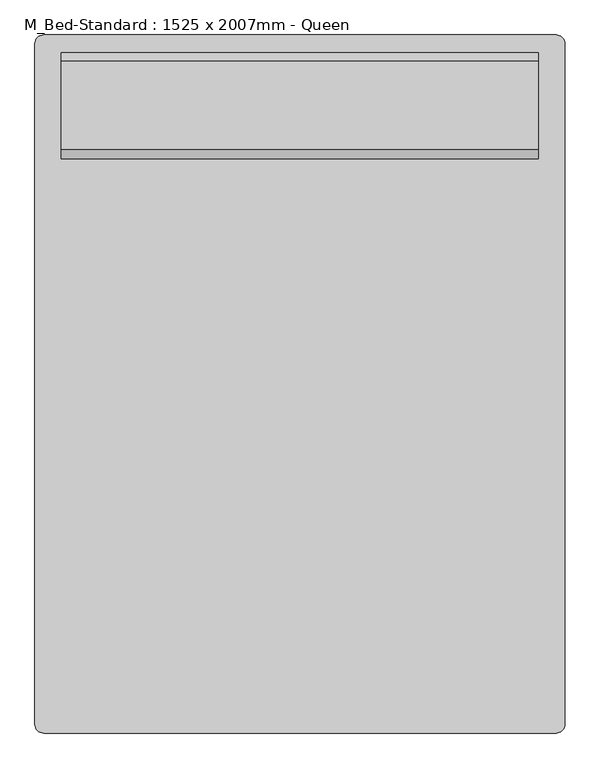
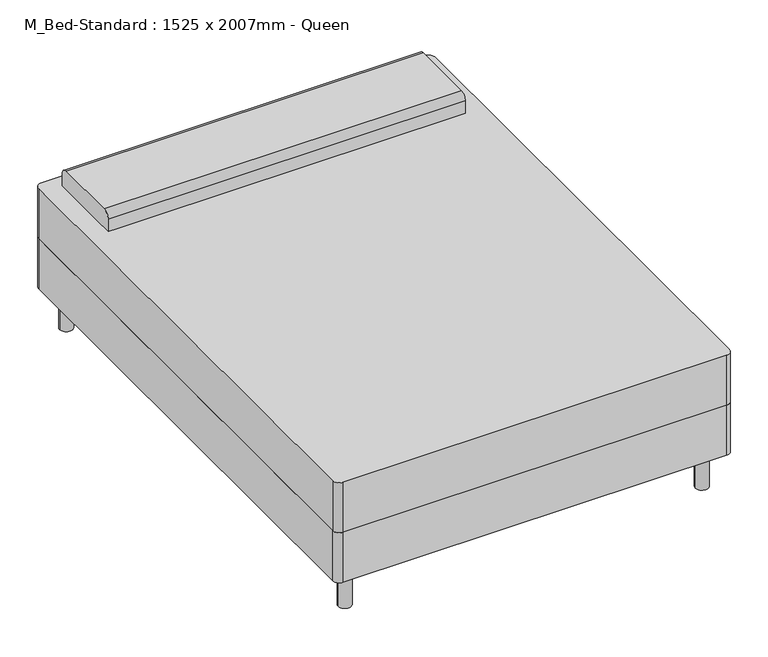
"""IFC4 building model written with IfcOpenShell, lengths in millimetres: furniture geometry, M_Bed-Standard : 1525 x 2007mm - Queen."""

from ifc_helpers import new_model, si_unit, point, frame, frame_2d, origin, origin_with_axes, place, context, project, spatial, polyline, circle_curve, trimmed, segment, composite_curve, outline, extrude, source, transform, mapped, element, save


def m_bed_standard_1525_x_2007mm_queen_67038778(model_context):
    return source(origin(), model_context, "Body", "SweptSolid", [
        extrude(outline(composite_curve([segment(polyline([(-491.0114754, -1023.695082), (-491.0114754, 932.504918)]), True, "CONTINUOUS"), segment(trimmed(circle_curve(frame_2d((-465.6114754, 932.504918)), 25.4), [point((-491.0114754, 932.504918))], [point((-465.6114754, 957.904918))], False, "CARTESIAN"), True, "CONTINUOUS"), segment(polyline([(-465.6114754, 957.904918), (1008.5885246, 957.904918)]), True, "CONTINUOUS"), segment(trimmed(circle_curve(frame_2d((1008.5885246, 932.504918)), 25.4), [point((1008.5885246, 957.904918))], [point((1033.9885246, 932.504918))], False, "CARTESIAN"), True, "CONTINUOUS"), segment(polyline([(1033.9885246, 932.504918), (1033.9885246, -1023.695082)]), True, "CONTINUOUS"), segment(trimmed(circle_curve(frame_2d((1008.5885246, -1023.695082)), 25.4), [point((1033.9885246, -1023.695082))], [point((1008.5885246, -1049.095082))], False, "CARTESIAN"), True, "CONTINUOUS"), segment(polyline([(1008.5885246, -1049.095082), (-465.6114754, -1049.095082)]), True, "CONTINUOUS"), segment(trimmed(circle_curve(frame_2d((-465.6114754, -1023.695082)), 25.4), [point((-465.6114754, -1049.095082))], [point((-491.0114754, -1023.695082))], False, "CARTESIAN"), True, "CONTINUOUS")], self_intersect=False)), frame((0.0, 0.0, 152.4), z_axis=(0.0, 0.0, 1.0), x_axis=(1.0, 0.0, 0.0)), (0.0, 0.0, 1.0), 203.2),
        extrude(outline(composite_curve([segment(polyline([(602.304918, 558.8), (602.304918, 609.6)]), True, "CONTINUOUS"), segment(trimmed(circle_curve(frame_2d((627.704918, 609.6)), 25.4), [point((602.304918, 609.6))], [point((627.704918, 635.0))], False, "CARTESIAN"), True, "CONTINUOUS"), segment(polyline([(627.704918, 635.0), (881.704918, 635.0)]), True, "CONTINUOUS"), segment(trimmed(circle_curve(frame_2d((881.704918, 609.6)), 25.4), [point((881.704918, 635.0))], [point((907.104918, 609.6))], False, "CARTESIAN"), True, "CONTINUOUS"), segment(polyline([(907.104918, 609.6), (907.104918, 558.8), (602.304918, 558.8)]), True, "CONTINUOUS")], self_intersect=False)), frame((-414.8114754, 0.0, 0.0), z_axis=(1.0, 0.0, 0.0), x_axis=(0.0, 1.0, 0.0)), (0.0, 0.0, 1.0), 1372.6),
        extrude(outline(composite_curve([segment(trimmed(circle_curve(frame_2d((-414.8114754, 881.704918)), 25.4), [point((-440.2114754, 881.704918))], [point((-389.4114754, 881.704918))], False, "CARTESIAN"), True, "CONTINUOUS"), segment(trimmed(circle_curve(frame_2d((-414.8114754, 881.704918)), 25.4), [point((-389.4114754, 881.704918))], [point((-440.2114754, 881.704918))], False, "CARTESIAN"), True, "CONTINUOUS")], self_intersect=False)), origin_with_axes(), (0.0, 0.0, 1.0), 152.4),
        extrude(outline(composite_curve([segment(trimmed(circle_curve(frame_2d((957.7885246, 881.704918)), 25.4), [point((932.3885246, 881.704918))], [point((983.1885246, 881.704918))], False, "CARTESIAN"), True, "CONTINUOUS"), segment(trimmed(circle_curve(frame_2d((957.7885246, 881.704918)), 25.4), [point((983.1885246, 881.704918))], [point((932.3885246, 881.704918))], False, "CARTESIAN"), True, "CONTINUOUS")], self_intersect=False)), origin_with_axes(), (0.0, 0.0, 1.0), 152.4),
        extrude(outline(composite_curve([segment(trimmed(circle_curve(frame_2d((957.7885246, -972.895082)), 25.4), [point((932.3885246, -972.895082))], [point((983.1885246, -972.895082))], False, "CARTESIAN"), True, "CONTINUOUS"), segment(trimmed(circle_curve(frame_2d((957.7885246, -972.895082)), 25.4), [point((983.1885246, -972.895082))], [point((932.3885246, -972.895082))], False, "CARTESIAN"), True, "CONTINUOUS")], self_intersect=False)), origin_with_axes(), (0.0, 0.0, 1.0), 152.4),
        extrude(outline(composite_curve([segment(trimmed(circle_curve(frame_2d((-414.8114754, -972.895082)), 25.4), [point((-440.2114754, -972.895082))], [point((-389.4114754, -972.895082))], False, "CARTESIAN"), True, "CONTINUOUS"), segment(trimmed(circle_curve(frame_2d((-414.8114754, -972.895082)), 25.4), [point((-389.4114754, -972.895082))], [point((-440.2114754, -972.895082))], False, "CARTESIAN"), True, "CONTINUOUS")], self_intersect=False)), origin_with_axes(), (0.0, 0.0, 1.0), 152.4),
        extrude(outline(composite_curve([segment(polyline([(-465.6114754, 957.904918), (1008.5885246, 957.904918)]), True, "CONTINUOUS"), segment(trimmed(circle_curve(frame_2d((1008.5885246, 932.504918)), 25.4), [point((1008.5885246, 957.904918))], [point((1033.9885246, 932.504918))], False, "CARTESIAN"), True, "CONTINUOUS"), segment(polyline([(1033.9885246, 932.504918), (1033.9885246, -1023.695082)]), True, "CONTINUOUS"), segment(trimmed(circle_curve(frame_2d((1008.5885246, -1023.695082)), 25.4), [point((1033.9885246, -1023.695082))], [point((1008.5885246, -1049.095082))], False, "CARTESIAN"), True, "CONTINUOUS"), segment(polyline([(1008.5885246, -1049.095082), (-465.6114754, -1049.095082)]), True, "CONTINUOUS"), segment(trimmed(circle_curve(frame_2d((-465.6114754, -1023.695082)), 25.4), [point((-465.6114754, -1049.095082))], [point((-491.0114754, -1023.695082))], False, "CARTESIAN"), True, "CONTINUOUS"), segment(polyline([(-491.0114754, -1023.695082), (-491.0114754, 932.504918)]), True, "CONTINUOUS"), segment(trimmed(circle_curve(frame_2d((-465.6114754, 932.504918)), 25.4), [point((-491.0114754, 932.504918))], [point((-465.6114754, 957.904918))], False, "CARTESIAN"), True, "CONTINUOUS")], self_intersect=False)), frame((0.0, 0.0, 355.6), z_axis=(0.0, 0.0, 1.0), x_axis=(1.0, 0.0, 0.0)), (0.0, 0.0, 1.0), 203.2),
    ])


if __name__ == "__main__":
    model = new_model("IFC4")
    model_context = context("Model", 3, world=origin())
    ifc_project = project(units=[si_unit("LENGTHUNIT", "METRE", prefix="MILLI")], contexts=[model_context])
    site = spatial("IfcSite", under=ifc_project)
    building = spatial("IfcBuilding", under=site)
    placement = place(None, origin())
    m_bed_standard_1525_x_2007mm_queen_shape = m_bed_standard_1525_x_2007mm_queen_67038778(model_context)
    element("IfcFurniture", 1, ObjectType="M_Bed-Standard : 1525 x 2007mm - Queen", at=placement, inside=building, context=model_context, shape_type="MappedRepresentation", body=[
        mapped(m_bed_standard_1525_x_2007mm_queen_shape, transform((0.0, 0.0, 0.0), x_axis=(1.0, 0.0, 0.0), y_axis=(0.0, 1.0, 0.0), z_axis=(0.0, 0.0, 1.0))),
    ])
    save(model, "model.ifc")

# Revit data of these elements
# Type "M_Bed-Standard : 1525 x 2007mm - Queen"
#   Manufacturer = "Manufacturer"
#   AccessibilityPerformance = "AccessibilityPerformance"
#   CodePerformance = "CodePerformance"
#   Area = "Area"
#   Color = "Color"
#   Constituents = "Constituents"
#   Features = "Features"
#   Finish = "Finish"
#   Grade = "Grade"
#   Material = "Material"
#   ModelReference = "ModelReference"
#   NominalHeight = "NominalHeight"
#   NominalLength = "NominalLength"
#   NominalWidth = "NominalWidth"
#   ProductionYear = "ProductionYear"
#   Reference = "Reference"
#   Shape = "Shape"
#   Size = "Size"
#   SustainabilityPerformance = "SustainabilityPerformance"
#   WarrantyDescription = "WarrantyDescription"
#   WarrantyDurationLabor = "WarrantyDurationLabor"
#   WarrantyDurationParts = "WarrantyDurationParts"
#   WarrantyGuarantorLabor = "WarrantyGuarantorLabor"
#   WarrantyGuarantorParts = "WarrantyGuarantorParts"
#   ExpectedLife = "ExpectedLife"
#   ReplacementCost = "ReplacementCost"
#   AssetAccountingType = "NONFIXED"
#   ModelLabel = "ModelLabel"
#   Length = 2.007 m
#   Width = 1.525 m
#   Leg Material = Metal - Chrome
#   Mattress Material = Textile - White
# Element 1 (IfcFurniture, "M_Bed-Standard : 1525 x 2007mm - Queen")
#   Materials on its faces: "Textile - White", "Metal - Chrome"
# Materials
#   "Metal - Chrome": class "Metal", colour RGB 17 17 17, transparency 0
#   "Textile - White": class "Fabric", colour RGB 247 247 239, transparency 0
